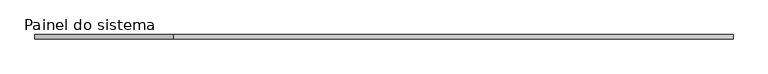
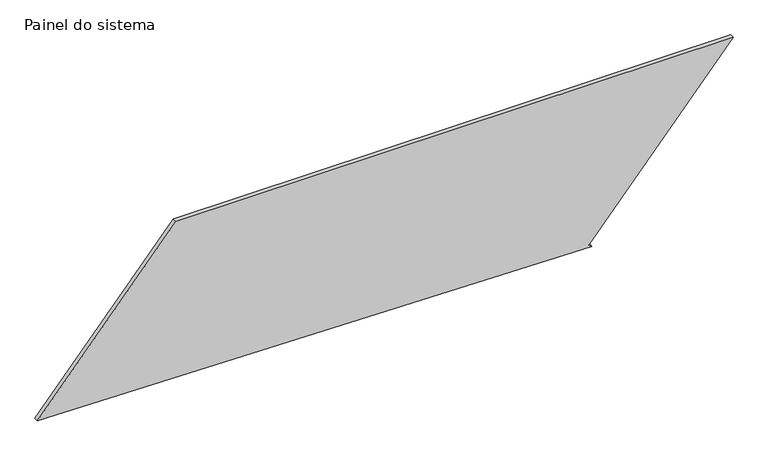
"""IFC4 building model written with IfcOpenShell, lengths in millimetres: plate geometry, Painel do sistema : Envidraçado."""

from ifc_helpers import new_model, si_unit, frame, origin, place, context, project, spatial, polyline, outline, extrude, source, transform, mapped, element, save


def painel_do_sistema_b7530998(model_context):
    return source(origin(), model_context, "Body", "SweptSolid", [
        extrude(outline(polyline([(0.0, 1242.4890976), (16.2242617, 1223.4687576), (1032.8985016, 2090.6871672), (1032.8985016, -1257.871482), (56.5559282, -2090.6871672), (0.0, 1242.4890976)])), frame((0.0, 24.5, 0.0), z_axis=(0.0, 1.0, 0.0), x_axis=(0.0, 0.0, 1.0)), (0.0, 0.0, 1.0), 25.0),
    ])


if __name__ == "__main__":
    model = new_model("IFC4")
    model_context = context("Model", 3, world=origin())
    ifc_project = project(units=[si_unit("LENGTHUNIT", "METRE", prefix="MILLI")], contexts=[model_context])
    site = spatial("IfcSite", under=ifc_project)
    building = spatial("IfcBuilding", under=site)
    placement = place(None, origin())
    painel_do_sistema_shape = painel_do_sistema_b7530998(model_context)
    element("IfcPlate", 1, ObjectType="Painel do sistema : Envidraçado", at=placement, inside=building, context=model_context, shape_type="MappedRepresentation", body=[
        mapped(painel_do_sistema_shape, transform((0.0, 0.0, 0.0), x_axis=(1.0, 0.0, 0.0), y_axis=(0.0, 1.0, 0.0), z_axis=(0.0, 0.0, 1.0))),
    ])
    save(model, "model.ifc")

# Revit data of these elements
# Type "Painel do sistema : Envidraçado"
#   Construction Type Id = "GSP4R"
#   Analytic Construction = "Vidraça única Pilkington 1/8 pol"
#   Visual Light Transmittance = 0.9
#   Solar Heat Gain Coefficient = 0.86
#   Heat Transfer Coefficient (U) = 6.7069 W/(m²·K)
# Element 1 (IfcPlate, "Painel do sistema : Envidraçado")
#   Materials on its faces: "Vidro"
# Materials
#   "Vidro": class "Vidro", colour RGB 0 128 192, transparency 0.9, Description = "Vidro de sílica", Cost = 0
